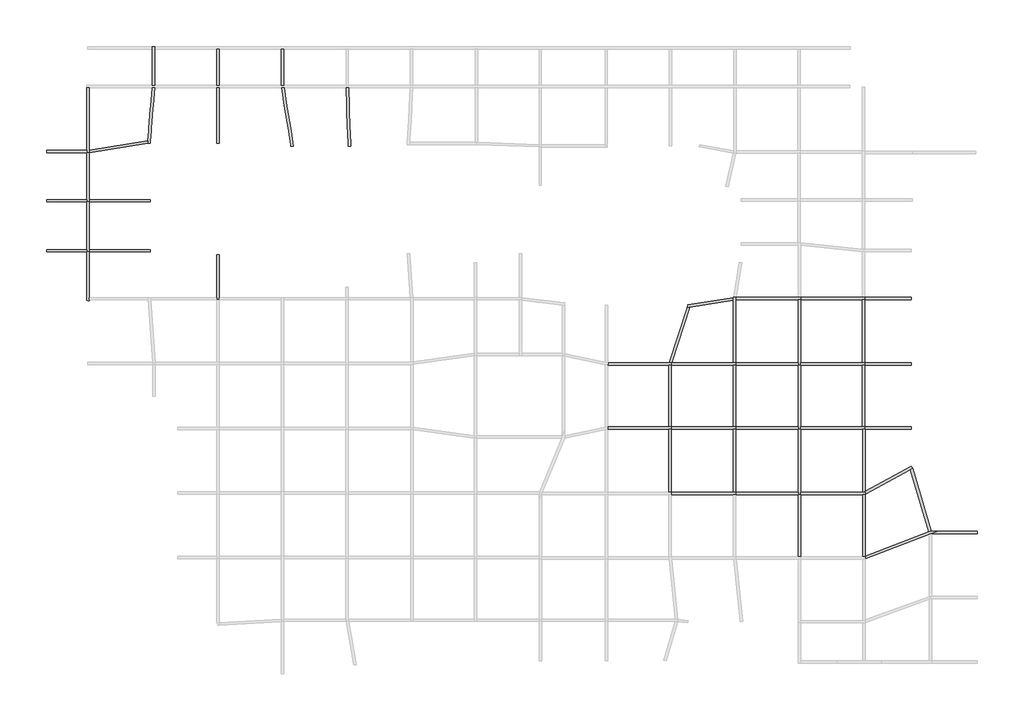
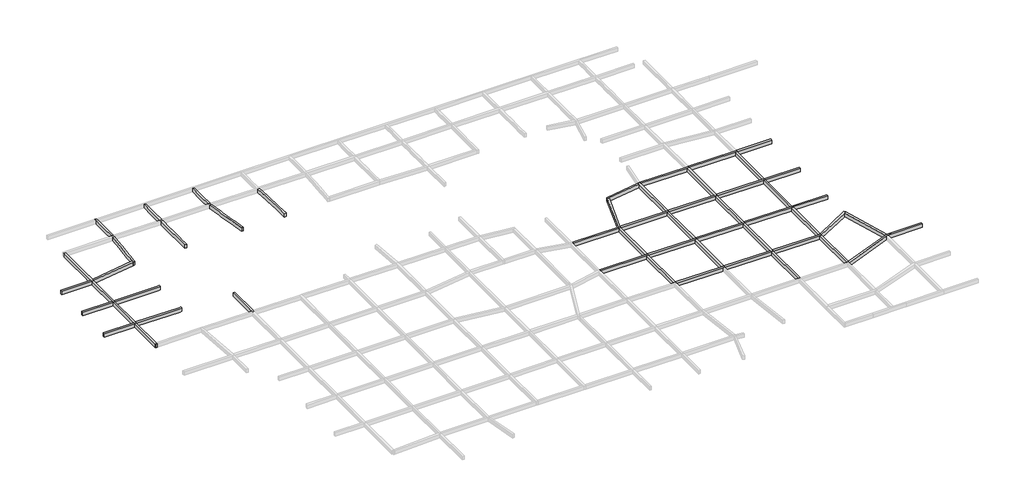
# One storey, part 6 of 8: 53 beams.
"""IFC4 building model written with IfcOpenShell, lengths in millimetres."""

from ifc_helpers import new_model, si_unit, frame, origin, place, context, project, spatial, polyline, outline, extrude, faceted_brep, element, save

model = new_model("IFC4")

# Units and contexts
model_context = context("Model", 3, world=origin())
ifc_project = project(units=[si_unit("LENGTHUNIT", "METRE", prefix="MILLI")], contexts=[model_context])

# Site, building, storey
site = spatial("IfcSite", under=ifc_project)
building = spatial("IfcBuilding", under=site)
storey = spatial("IfcBuildingStorey", under=building, Name="层高", Elevation=3300.0)

# Beams
placement = place(None, origin())
element("IfcBeam", 1, ObjectType="混凝土 - 矩形梁 : KL_beam", at=placement, inside=storey, context=model_context, shape_type="Brep", body=[
    faceted_brep([(62108.8476291, 145017.045189, 3300.0), (62408.8476291, 145017.045189, 3300.0), (62408.8476291, 145038.9496025, 3300.0), (62408.8476291, 145342.6952689, 3300.0), (62408.8476291, 147654.2446479, 3300.0), (62408.8476291, 148054.2446479, 3300.0), (62408.8476291, 150406.6496336, 3300.0), (62408.8476291, 150806.6496336, 3300.0), (62408.8476291, 152967.0451916, 3300.0), (62108.8476291, 152967.0451916, 3300.0), (62108.8476291, 145317.045189, 3300.0), (62108.8476291, 145017.045189, 2700.0), (62108.8476291, 152967.0451916, 2700.0), (62108.8476291, 150806.6496336, 2700.0), (62108.8476291, 150406.6496336, 2700.0), (62108.8476291, 148054.2446479, 2700.0), (62108.8476291, 147654.2446479, 2700.0), (62108.8476291, 145317.045189, 2700.0), (62408.8476291, 145017.045189, 2700.0), (62408.8476291, 152967.0451916, 2700.0), (62408.8476291, 150806.6496336, 2700.0), (62408.8476291, 150406.6496336, 2700.0), (62408.8476291, 148054.2446479, 2700.0), (62408.8476291, 147654.2446479, 2700.0), (62408.8476291, 145342.6952689, 2700.0), (62408.8476291, 145038.9496025, 2700.0)], [[[0, 1, 2, 3, 4, 5, 6, 7, 8, 9, 10]], [[11, 0, 10, 9, 12, 13, 14, 15, 16, 17]], [[18, 11, 17, 16, 15, 14, 13, 12, 19, 20, 21, 22, 23, 24, 25]], [[1, 18, 25, 24, 23, 22, 21, 20, 19, 8, 7, 6, 5, 4, 3, 2]], [[9, 8, 19, 12]], [[1, 0, 11, 18]]]),
])
element("IfcBeam", 2, ObjectType="混凝土 - 矩形梁 : KL_beam", at=placement, inside=storey, context=model_context, shape_type="SweptSolid", body=[
    extrude(outline(polyline([(57170.338145, 145017.045189), (57170.338145, 145317.045189), (62108.8476291, 145317.045189), (62108.8476291, 145017.045189), (57170.338145, 145017.045189)])), frame((0.0, 0.0, 2700.0), z_axis=(0.0, 0.0, 1.0), x_axis=(1.0, 0.0, 0.0)), (0.0, 0.0, 1.0), 600.0),
])
element("IfcBeam", 3, ObjectType="混凝土 - 矩形梁 : KL_beam", at=placement, inside=storey, context=model_context, shape_type="Brep", body=[
    faceted_brep([(62108.8476291, 139017.045189, 3300.0), (62408.8476291, 139017.045189, 3300.0), (62408.8476291, 139317.045189, 3300.0), (62408.8476291, 145017.045189, 3300.0), (62108.8476291, 145017.045189, 3300.0), (62108.8476291, 139317.045189, 3300.0), (62108.8476291, 139017.045189, 2700.0), (62108.8476291, 145017.045189, 2700.0), (62108.8476291, 139317.045189, 2700.0), (62408.8476291, 139017.045189, 2700.0), (62408.8476291, 145017.045189, 2700.0), (62408.8476291, 139317.045189, 2700.0)], [[[0, 1, 2, 3, 4, 5]], [[6, 0, 5, 4, 7, 8]], [[9, 6, 8, 7, 10, 11]], [[1, 9, 11, 10, 3, 2]], [[4, 3, 10, 7]], [[1, 0, 6, 9]]]),
])
element("IfcBeam", 4, ObjectType="混凝土 - 矩形梁 : KL_beam", at=placement, inside=storey, context=model_context, shape_type="Brep", body=[
    faceted_brep([(62108.8476291, 132904.2446453, 3300.0), (62408.8476291, 132904.2446453, 3300.0), (62408.8476291, 133204.2446453, 3300.0), (62408.8476291, 139017.045189, 3300.0), (62108.8476291, 139017.045189, 3300.0), (62108.8476291, 133204.2446453, 3300.0), (62108.8476291, 132904.2446453, 2700.0), (62108.8476291, 139017.045189, 2700.0), (62108.8476291, 133204.2446453, 2700.0), (62408.8476291, 132904.2446453, 2700.0), (62408.8476291, 139017.045189, 2700.0), (62408.8476291, 133204.2446453, 2700.0)], [[[0, 1, 2, 3, 4, 5]], [[6, 0, 5, 4, 7, 8]], [[9, 6, 8, 7, 10, 11]], [[1, 9, 11, 10, 3, 2]], [[1, 0, 6, 9]], [[4, 3, 10, 7]]]),
])
element("IfcBeam", 5, ObjectType="混凝土 - 矩形梁 : KL_beam", at=placement, inside=storey, context=model_context, shape_type="Brep", body=[
    faceted_brep([(62408.8476291, 126967.1449171, 2700.0), (62408.8476291, 126967.1449171, 3300.0), (62233.8430954, 126967.1449171, 3300.0), (62233.8430954, 126967.1449171, 2700.0), (62108.8476291, 127027.0451941, 3300.0), (62113.8430954, 127027.0451941, 3300.0), (62233.8430954, 127027.0451941, 3300.0), (62408.8476291, 127035.802002, 3300.0), (62408.8476291, 127335.802002, 3300.0), (62408.8476291, 132904.2446453, 3300.0), (62108.8476291, 132904.2446453, 3300.0), (62108.8476291, 127027.0451941, 2700.0), (62108.8476291, 132904.2446453, 2700.0), (62233.8430954, 127027.0451941, 2700.0), (62408.8476291, 132904.2446453, 2700.0), (62408.8476291, 127335.802002, 2700.0), (62408.8476291, 127035.802002, 2700.0)], [[[0, 1, 2, 3]], [[4, 5, 6, 2, 1, 7, 8, 9, 10]], [[11, 4, 10, 12]], [[13, 11, 12, 14, 15, 16, 0, 3]], [[1, 0, 16, 15, 14, 9, 8, 7]], [[4, 11, 13, 6, 5]], [[6, 13, 3, 2]], [[10, 9, 14, 12]]]),
])
element("IfcBeam", 6, ObjectType="混凝土 - 矩形梁 : KL_beam", at=placement, inside=storey, context=model_context, shape_type="SweptSolid", body=[
    extrude(outline(polyline([(57170.338145, 132904.2446453), (57170.338145, 133204.2446453), (62108.8476291, 133204.2446453), (62108.8476291, 132904.2446453), (57170.338145, 132904.2446453)])), frame((0.0, 0.0, 2700.0), z_axis=(0.0, 0.0, 1.0), x_axis=(1.0, 0.0, 0.0)), (0.0, 0.0, 1.0), 600.0),
])
element("IfcBeam", 7, ObjectType="混凝土 - 矩形梁 : KL_beam", at=placement, inside=storey, context=model_context, shape_type="SweptSolid", body=[
    extrude(outline(polyline([(57170.338145, 139017.045189), (57170.338145, 139317.045189), (62108.8476291, 139317.045189), (62108.8476291, 139017.045189), (57170.338145, 139017.045189)])), frame((0.0, 0.0, 2700.0), z_axis=(0.0, 0.0, 1.0), x_axis=(1.0, 0.0, 0.0)), (0.0, 0.0, 1.0), 600.0),
])
element("IfcBeam", 8, ObjectType="混凝土 - 矩形梁 : KL_beam", at=placement, inside=storey, context=model_context, shape_type="Brep", body=[
    faceted_brep([(70393.6976621, 158016.4462381, 3300.0), (70393.6976621, 158016.4462381, 2700.0), (70093.6976621, 158016.4462381, 2700.0), (70093.6976621, 158016.4462381, 3300.0), (70093.6976621, 158006.8472847, 3300.0), (70093.6976621, 157706.8472847, 3300.0), (70093.6976621, 155766.9462381, 3300.0), (70093.6976621, 155366.9462381, 3300.0), (70093.6976621, 153267.0451916, 3300.0), (70393.6976621, 153267.0451916, 3300.0), (70393.6976621, 155366.9462381, 3300.0), (70393.6976621, 155766.9462381, 3300.0), (70393.6976621, 157706.8472847, 3300.0), (70393.6976621, 158006.8472847, 3300.0), (70093.6976621, 158006.8472847, 2700.0), (70093.6976621, 157706.8472847, 2700.0), (70093.6976621, 155766.9462381, 2700.0), (70093.6976621, 155366.9462381, 2700.0), (70093.6976621, 153267.0451916, 2700.0), (70393.6976621, 158006.8472847, 2700.0), (70393.6976621, 157706.8472847, 2700.0), (70393.6976621, 155766.9462381, 2700.0), (70393.6976621, 155366.9462381, 2700.0), (70393.6976621, 153267.0451916, 2700.0)], [[[0, 1, 2, 3]], [[0, 3, 4, 5, 6, 7, 8, 9, 10, 11, 12, 13]], [[3, 2, 14, 15, 16, 17, 18, 8, 7, 6, 5, 4]], [[2, 1, 19, 20, 21, 22, 23, 18, 17, 16, 15, 14]], [[1, 0, 13, 12, 11, 10, 9, 23, 22, 21, 20, 19]], [[9, 8, 18, 23]]]),
])
element("IfcBeam", 9, ObjectType="混凝土 - 矩形梁 : KL_beam", at=placement, inside=storey, context=model_context, shape_type="Brep", body=[
    faceted_brep([(77972.7452463, 153267.0451916, 3300.0), (78272.7452463, 153267.0451916, 3300.0), (78272.7452463, 155366.9462381, 3300.0), (78272.7452463, 155766.9462381, 3300.0), (78272.7452463, 157706.8472847, 3300.0), (77972.7452463, 157706.8472847, 3300.0), (77972.7452463, 155766.9462381, 3300.0), (77972.7452463, 155366.9462381, 3300.0), (77972.7452463, 153267.0451916, 2700.0), (77972.7452463, 157706.8472847, 2700.0), (77972.7452463, 155766.9462381, 2700.0), (77972.7452463, 155366.9462381, 2700.0), (78272.7452463, 153267.0451916, 2700.0), (78272.7452463, 157706.8472847, 2700.0), (78272.7452463, 155766.9462381, 2700.0), (78272.7452463, 155366.9462381, 2700.0)], [[[0, 1, 2, 3, 4, 5, 6, 7]], [[8, 0, 7, 6, 5, 9, 10, 11]], [[12, 8, 11, 10, 9, 13, 14, 15]], [[1, 12, 15, 14, 13, 4, 3, 2]], [[1, 0, 8, 12]], [[5, 4, 13, 9]]]),
])
element("IfcBeam", 10, ObjectType="混凝土 - 矩形梁 : KL_beam", at=placement, inside=storey, context=model_context, shape_type="Brep", body=[
    faceted_brep([(85892.7452463, 153267.0451916, 3300.0), (86192.7452463, 153267.0451916, 3300.0), (86192.7452463, 155366.9462381, 3300.0), (86192.7452463, 155766.9462381, 3300.0), (86192.7452463, 157706.8472847, 3300.0), (85892.7452463, 157706.8472847, 3300.0), (85892.7452463, 155766.9462381, 3300.0), (85892.7452463, 155366.9462381, 3300.0), (85892.7452463, 153267.0451916, 2700.0), (85892.7452463, 157706.8472847, 2700.0), (85892.7452463, 155766.9462381, 2700.0), (85892.7452463, 155366.9462381, 2700.0), (86192.7452463, 153267.0451916, 2700.0), (86192.7452463, 157706.8472847, 2700.0), (86192.7452463, 155766.9462381, 2700.0), (86192.7452463, 155366.9462381, 2700.0)], [[[0, 1, 2, 3, 4, 5, 6, 7]], [[8, 0, 7, 6, 5, 9, 10, 11]], [[12, 8, 11, 10, 9, 13, 14, 15]], [[1, 12, 15, 14, 13, 4, 3, 2]], [[1, 0, 8, 12]], [[5, 4, 13, 9]]]),
])
element("IfcBeam", 11, ObjectType="混凝土 - 矩形梁 : KL_beam", at=placement, inside=storey, context=model_context, shape_type="Brep", body=[
    faceted_brep([(69518.4633077, 146165.9301761, 3300.0), (69533.6976621, 146168.3450494, 3300.0), (69695.5125279, 146193.9951293, 3300.0), (69823.484619, 146214.2806226, 3300.0), (69846.6115888, 146493.9951293, 3300.0), (69942.541742, 147654.2446479, 3300.0), (69975.6139913, 148054.2446479, 3300.0), (70170.1123015, 150406.6496336, 3300.0), (70203.1845508, 150806.6496336, 3300.0), (70381.8074018, 152967.0451916, 3300.0), (70080.7837355, 152967.0451916, 3300.0), (69902.1608844, 150806.6496336, 3300.0), (69869.0886352, 150406.6496336, 3300.0), (69674.590325, 148054.2446479, 3300.0), (69641.5180757, 147654.2446479, 3300.0), (69543.9107052, 146473.7096361, 3300.0), (69518.4633077, 146165.9301761, 2700.0), (70080.7837355, 152967.0451916, 2700.0), (69902.1608844, 150806.6496336, 2700.0), (69869.0886352, 150406.6496336, 2700.0), (69674.590325, 148054.2446479, 2700.0), (69641.5180757, 147654.2446479, 2700.0), (69543.9107052, 146473.7096361, 2700.0), (69823.484619, 146214.2806226, 2700.0), (69695.5125279, 146193.9951293, 2700.0), (69533.6976621, 146168.3450494, 2700.0), (70381.8074018, 152967.0451916, 2700.0), (70203.1845508, 150806.6496336, 2700.0), (70170.1123015, 150406.6496336, 2700.0), (69975.6139913, 148054.2446479, 2700.0), (69942.541742, 147654.2446479, 2700.0), (69846.6115888, 146493.9951293, 2700.0)], [[[0, 1, 2, 3, 4, 5, 6, 7, 8, 9, 10, 11, 12, 13, 14, 15]], [[16, 0, 15, 14, 13, 12, 11, 10, 17, 18, 19, 20, 21, 22]], [[23, 24, 25, 16, 22, 21, 20, 19, 18, 17, 26, 27, 28, 29, 30, 31]], [[3, 23, 31, 30, 29, 28, 27, 26, 9, 8, 7, 6, 5, 4]], [[10, 9, 26, 17]], [[3, 2, 1, 0, 16, 25, 24, 23]]]),
])
element("IfcBeam", 12, ObjectType="混凝土 - 矩形梁 : KL_beam", at=placement, inside=storey, context=model_context, shape_type="Brep", body=[
    faceted_brep([(62408.8476291, 145342.6952689, 2700.0), (62408.8476291, 145342.6952689, 3300.0), (69543.9107052, 146473.7096361, 3300.0), (69543.9107052, 146473.7096361, 2700.0), (62408.8476291, 145317.045189, 2700.0), (62408.8476291, 145038.9496025, 2700.0), (62408.8476291, 145038.9496025, 3300.0), (62408.8476291, 145317.045189, 3300.0), (69518.4633077, 146165.9301761, 3300.0), (69518.4633077, 146165.9301761, 2700.0)], [[[0, 1, 2, 3]], [[1, 0, 4, 5, 6, 7]], [[7, 6, 8, 2, 1]], [[4, 0, 3, 9, 5]], [[6, 5, 9, 8]], [[3, 2, 8, 9]]]),
])
element("IfcBeam", 13, ObjectType="混凝土 - 矩形梁 : KL_beam", at=placement, inside=storey, context=model_context, shape_type="Brep", body=[
    faceted_brep([(69858.8476291, 139317.045189, 3300.0), (69858.8476291, 139017.045189, 3300.0), (69858.8476291, 139017.045189, 2700.0), (69858.8476291, 139317.045189, 2700.0), (69833.6976621, 139317.045189, 3300.0), (69533.6976621, 139317.045189, 3300.0), (62408.8476291, 139317.045189, 3300.0), (62408.8476291, 139017.045189, 3300.0), (69533.6976621, 139017.045189, 3300.0), (69833.6976621, 139017.045189, 3300.0), (62408.8476291, 139017.045189, 2700.0), (69533.6976621, 139017.045189, 2700.0), (69833.6976621, 139017.045189, 2700.0), (62408.8476291, 139317.045189, 2700.0), (69533.6976621, 139317.045189, 2700.0), (69833.6976621, 139317.045189, 2700.0)], [[[0, 1, 2, 3]], [[1, 0, 4, 5, 6, 7, 8, 9]], [[2, 1, 9, 8, 7, 10, 11, 12]], [[3, 2, 12, 11, 10, 13, 14, 15]], [[0, 3, 15, 14, 13, 6, 5, 4]], [[7, 6, 13, 10]]]),
])
element("IfcBeam", 14, ObjectType="混凝土 - 矩形梁 : KL_beam", at=placement, inside=storey, context=model_context, shape_type="Brep", body=[
    faceted_brep([(69833.6976621, 132904.2446453, 3300.0), (69833.6976621, 133204.2446453, 3300.0), (69533.6976621, 133204.2446453, 3300.0), (62408.8476291, 133204.2446453, 3300.0), (62408.8476291, 132904.2446453, 3300.0), (69535.8470854, 132904.2446453, 3300.0), (69833.6976621, 132904.2446453, 2700.0), (62408.8476291, 132904.2446453, 2700.0), (69535.8470854, 132904.2446453, 2700.0), (69833.6976621, 133204.2446453, 2700.0), (62408.8476291, 133204.2446453, 2700.0), (69533.6976621, 133204.2446453, 2700.0)], [[[0, 1, 2, 3, 4, 5]], [[6, 0, 5, 4, 7, 8]], [[9, 6, 8, 7, 10, 11]], [[1, 9, 11, 10, 3, 2]], [[4, 3, 10, 7]], [[1, 0, 6, 9]]]),
])
element("IfcBeam", 15, ObjectType="混凝土 - 矩形梁 : KL_beam", at=placement, inside=storey, context=model_context, shape_type="Brep", body=[
    faceted_brep([(78292.6046485, 132543.8985649, 3300.0), (78292.6046485, 132543.8985649, 2700.0), (77992.6046485, 132543.8985649, 2700.0), (77992.6046485, 132543.8985649, 3300.0), (77992.6046485, 127335.802002, 3300.0), (77992.6046485, 127035.802002, 3300.0), (78270.8225114, 127035.802002, 3300.0), (78292.6046485, 127035.802002, 3300.0), (78292.6046485, 127335.802002, 3300.0), (77992.6046485, 127335.802002, 2700.0), (77992.6046485, 127035.802002, 2700.0), (78292.6046485, 127335.802002, 2700.0), (78292.6046485, 127035.802002, 2700.0), (78270.8225114, 127035.802002, 2700.0)], [[[0, 1, 2, 3]], [[0, 3, 4, 5, 6, 7, 8]], [[3, 2, 9, 10, 5, 4]], [[2, 1, 11, 12, 13, 10, 9]], [[1, 0, 8, 7, 12, 11]], [[7, 6, 5, 10, 13, 12]]]),
])
element("IfcBeam", 16, ObjectType="混凝土 - 矩形梁 : KL_beam", at=placement, inside=storey, context=model_context, shape_type="Brep", body=[
    faceted_brep([(125748.8238726, 111515.2247274, 3300.0), (125748.8238726, 111243.7571224, 3300.0), (125748.8238726, 111215.2247274, 3300.0), (133248.8238805, 111215.2247274, 3300.0), (133548.8238805, 111215.2247274, 3300.0), (133548.8238805, 111515.2247274, 3300.0), (133248.8238805, 111515.2247274, 3300.0), (133548.8238805, 111215.2247274, 2700.0), (125748.8238726, 111215.2247274, 2700.0), (133248.8238805, 111215.2247274, 2700.0), (125748.8238726, 111243.7571224, 2700.0), (125748.8238726, 111515.2247274, 2700.0), (133248.8238805, 111515.2247274, 2700.0), (133548.8238805, 111515.2247274, 2700.0)], [[[0, 1, 2, 3, 4, 5, 6]], [[7, 4, 3, 2, 8, 9]], [[8, 10, 11, 12, 13, 7, 9]], [[11, 0, 6, 5, 13, 12]], [[0, 11, 10, 8, 2, 1]], [[5, 4, 7, 13]]]),
])
element("IfcBeam", 17, ObjectType="混凝土 - 矩形梁 : KL_beam", at=placement, inside=storey, context=model_context, shape_type="Brep", body=[
    faceted_brep([(125814.5895158, 119344.1147453, 3300.0), (125783.0582452, 119044.1147453, 3300.0), (133248.8238805, 119044.1147453, 3300.0), (133548.8238805, 119044.1147453, 3300.0), (133548.8238805, 119344.1147453, 3300.0), (133289.6573621, 119344.1147453, 3300.0), (125783.0582452, 119044.1147453, 2700.0), (133248.8238805, 119044.1147453, 2700.0), (133548.8238805, 119044.1147453, 2700.0), (125814.5895158, 119344.1147453, 2700.0), (133289.6573621, 119344.1147453, 2700.0), (133548.8238805, 119344.1147453, 2700.0)], [[[0, 1, 2, 3, 4, 5]], [[1, 6, 7, 8, 3, 2]], [[6, 9, 10, 11, 8, 7]], [[9, 0, 5, 4, 11, 10]], [[0, 9, 6, 1]], [[4, 3, 8, 11]]]),
])
element("IfcBeam", 18, ObjectType="混凝土 - 矩形梁 : KL_beam", at=placement, inside=storey, context=model_context, shape_type="SweptSolid", body=[
    extrude(outline(polyline([(133548.8238805, 111515.2247274), (133248.8238805, 111515.2247274), (133248.8238805, 119044.1147453), (133548.8238805, 119044.1147453), (133548.8238805, 111515.2247274)])), frame((0.0, 0.0, 2700.0), z_axis=(0.0, 0.0, 1.0), x_axis=(1.0, 0.0, 0.0)), (0.0, 0.0, 1.0), 600.0),
])
element("IfcBeam", 19, ObjectType="混凝土 - 矩形梁 : KL_beam", at=placement, inside=storey, context=model_context, shape_type="SweptSolid", body=[
    extrude(outline(polyline([(133548.8238805, 103531.7102801), (133248.8238805, 103531.7102801), (133248.8238805, 111215.2247274), (133548.8238805, 111215.2247274), (133548.8238805, 103531.7102801)])), frame((0.0, 0.0, 2700.0), z_axis=(0.0, 0.0, 1.0), x_axis=(1.0, 0.0, 0.0)), (0.0, 0.0, 1.0), 600.0),
])
element("IfcBeam", 20, ObjectType="混凝土 - 矩形梁 : KL_beam", at=placement, inside=storey, context=model_context, shape_type="Brep", body=[
    faceted_brep([(141448.8238805, 119044.1147453, 3300.0), (141448.8238805, 119344.1147453, 3300.0), (141148.8238805, 119344.1147453, 3300.0), (133604.9310307, 119344.1147453, 3300.0), (133548.8238805, 119344.1147453, 3300.0), (133548.8238805, 119044.1147453, 3300.0), (141148.8238805, 119044.1147453, 3300.0), (141448.8238805, 119044.1147453, 2700.0), (133548.8238805, 119044.1147453, 2700.0), (141148.8238805, 119044.1147453, 2700.0), (141448.8238805, 119344.1147453, 2700.0), (133548.8238805, 119344.1147453, 2700.0), (133604.9310307, 119344.1147453, 2700.0), (141148.8238805, 119344.1147453, 2700.0)], [[[0, 1, 2, 3, 4, 5, 6]], [[7, 0, 6, 5, 8, 9]], [[10, 7, 9, 8, 11, 12, 13]], [[1, 10, 13, 12, 11, 4, 3, 2]], [[5, 4, 11, 8]], [[1, 0, 7, 10]]]),
])
element("IfcBeam", 21, ObjectType="混凝土 - 矩形梁 : KL_beam", at=placement, inside=storey, context=model_context, shape_type="Brep", body=[
    faceted_brep([(141448.8238805, 111215.2247274, 3300.0), (141448.8238805, 111515.2247274, 3300.0), (141148.8238805, 111515.2247274, 3300.0), (133548.8238805, 111515.2247274, 3300.0), (133548.8238805, 111215.2247274, 3300.0), (141148.8238805, 111215.2247274, 3300.0), (141448.8238805, 111215.2247274, 2700.0), (133548.8238805, 111215.2247274, 2700.0), (141148.8238805, 111215.2247274, 2700.0), (141448.8238805, 111515.2247274, 2700.0), (133548.8238805, 111515.2247274, 2700.0), (141148.8238805, 111515.2247274, 2700.0)], [[[0, 1, 2, 3, 4, 5]], [[6, 0, 5, 4, 7, 8]], [[9, 6, 8, 7, 10, 11]], [[1, 9, 11, 10, 3, 2]], [[4, 3, 10, 7]], [[1, 0, 6, 9]]]),
])
element("IfcBeam", 22, ObjectType="混凝土 - 矩形梁 : KL_beam", at=placement, inside=storey, context=model_context, shape_type="Brep", body=[
    faceted_brep([(141448.8238805, 103231.7102801, 3300.0), (141448.8238805, 103531.7102801, 3300.0), (141148.8238805, 103531.7102801, 3300.0), (133548.8238805, 103531.7102801, 3300.0), (133548.8238805, 103231.7102801, 3300.0), (141148.8238805, 103231.7102801, 3300.0), (141448.8238805, 103231.7102801, 2700.0), (133548.8238805, 103231.7102801, 2700.0), (141148.8238805, 103231.7102801, 2700.0), (141448.8238805, 103531.7102801, 2700.0), (133548.8238805, 103531.7102801, 2700.0), (141148.8238805, 103531.7102801, 2700.0)], [[[0, 1, 2, 3, 4, 5]], [[6, 0, 5, 4, 7, 8]], [[9, 6, 8, 7, 10, 11]], [[1, 9, 11, 10, 3, 2]], [[4, 3, 10, 7]], [[1, 0, 6, 9]]]),
])
element("IfcBeam", 23, ObjectType="混凝土 - 矩形梁 : KL_beam", at=placement, inside=storey, context=model_context, shape_type="SweptSolid", body=[
    extrude(outline(polyline([(141148.8238805, 111215.2247274), (141448.8238805, 111215.2247274), (141448.8238805, 103531.7102801), (141148.8238805, 103531.7102801), (141148.8238805, 111215.2247274)])), frame((0.0, 0.0, 2700.0), z_axis=(0.0, 0.0, 1.0), x_axis=(1.0, 0.0, 0.0)), (0.0, 0.0, 1.0), 600.0),
])
element("IfcBeam", 24, ObjectType="混凝土 - 矩形梁 : KL_beam", at=placement, inside=storey, context=model_context, shape_type="SweptSolid", body=[
    extrude(outline(polyline([(141148.8238805, 119044.1147453), (141448.8238805, 119044.1147453), (141448.8238805, 111515.2247274), (141148.8238805, 111515.2247274), (141148.8238805, 119044.1147453)])), frame((0.0, 0.0, 2700.0), z_axis=(0.0, 0.0, 1.0), x_axis=(1.0, 0.0, 0.0)), (0.0, 0.0, 1.0), 600.0),
])
element("IfcBeam", 25, ObjectType="混凝土 - 矩形梁 : KL_beam", at=placement, inside=storey, context=model_context, shape_type="Brep", body=[
    faceted_brep([(141448.8238805, 127344.1147453, 3300.0), (141170.7117777, 127344.1147453, 3300.0), (141148.8238805, 127344.1147453, 3300.0), (141148.8238805, 127321.9986816, 3300.0), (141148.8238805, 127205.9200013, 3300.0), (141148.8238805, 127018.1739614, 3300.0), (141148.8238805, 119344.1147453, 3300.0), (141448.8238805, 119344.1147453, 3300.0), (141448.8238805, 127044.1147453, 3300.0), (141448.8238805, 127344.1147453, 2700.0), (141448.8238805, 119344.1147453, 2700.0), (141448.8238805, 127044.1147453, 2700.0), (141148.8238805, 127344.1147453, 2700.0), (141170.7117777, 127344.1147453, 2700.0), (141148.8238805, 119344.1147453, 2700.0), (141148.8238805, 127018.1739614, 2700.0), (141148.8238805, 127205.9200013, 2700.0), (141148.8238805, 127321.9986816, 2700.0)], [[[0, 1, 2, 3, 4, 5, 6, 7, 8]], [[9, 0, 8, 7, 10, 11]], [[12, 13, 9, 11, 10, 14, 15, 16, 17]], [[2, 12, 17, 16, 15, 14, 6, 5, 4, 3]], [[7, 6, 14, 10]], [[2, 1, 0, 9, 13, 12]]]),
])
element("IfcBeam", 26, ObjectType="混凝土 - 矩形梁 : KL_beam", at=placement, inside=storey, context=model_context, shape_type="Brep", body=[
    faceted_brep([(149348.8238805, 127044.1147453, 3300.0), (149348.8238805, 127344.1147453, 3300.0), (149048.8238805, 127344.1147453, 3300.0), (141474.4513154, 127344.1147453, 3300.0), (141448.8238805, 127344.1147453, 3300.0), (141448.8238805, 127044.1147453, 3300.0), (149048.8238805, 127044.1147453, 3300.0), (149348.8238805, 127044.1147453, 2700.0), (141448.8238805, 127044.1147453, 2700.0), (149048.8238805, 127044.1147453, 2700.0), (149348.8238805, 127344.1147453, 2700.0), (141448.8238805, 127344.1147453, 2700.0), (141474.4513154, 127344.1147453, 2700.0), (149048.8238805, 127344.1147453, 2700.0)], [[[0, 1, 2, 3, 4, 5, 6]], [[7, 0, 6, 5, 8, 9]], [[10, 7, 9, 8, 11, 12, 13]], [[1, 10, 13, 12, 11, 4, 3, 2]], [[5, 4, 11, 8]], [[1, 0, 7, 10]]]),
])
element("IfcBeam", 27, ObjectType="混凝土 - 矩形梁 : KL_beam", at=placement, inside=storey, context=model_context, shape_type="Brep", body=[
    faceted_brep([(149048.8238805, 119044.1147453, 3300.0), (149348.8238805, 119044.1147453, 3300.0), (149348.8238805, 119344.1147453, 3300.0), (149348.8238805, 127044.1147453, 3300.0), (149048.8238805, 127044.1147453, 3300.0), (149048.8238805, 119344.1147453, 3300.0), (149048.8238805, 119044.1147453, 2700.0), (149048.8238805, 127044.1147453, 2700.0), (149048.8238805, 119344.1147453, 2700.0), (149348.8238805, 119044.1147453, 2700.0), (149348.8238805, 127044.1147453, 2700.0), (149348.8238805, 119344.1147453, 2700.0)], [[[0, 1, 2, 3, 4, 5]], [[6, 0, 5, 4, 7, 8]], [[9, 6, 8, 7, 10, 11]], [[1, 9, 11, 10, 3, 2]], [[4, 3, 10, 7]], [[1, 0, 6, 9]]]),
])
element("IfcBeam", 28, ObjectType="混凝土 - 矩形梁 : KL_beam", at=placement, inside=storey, context=model_context, shape_type="Brep", body=[
    faceted_brep([(149048.8238805, 111215.2247274, 3300.0), (149348.8238805, 111215.2247274, 3300.0), (149348.8238805, 111515.2247274, 3300.0), (149348.8238805, 119044.1147453, 3300.0), (149048.8238805, 119044.1147453, 3300.0), (149048.8238805, 111515.2247274, 3300.0), (149048.8238805, 111215.2247274, 2700.0), (149048.8238805, 119044.1147453, 2700.0), (149048.8238805, 111515.2247274, 2700.0), (149348.8238805, 111215.2247274, 2700.0), (149348.8238805, 119044.1147453, 2700.0), (149348.8238805, 111515.2247274, 2700.0)], [[[0, 1, 2, 3, 4, 5]], [[6, 0, 5, 4, 7, 8]], [[9, 6, 8, 7, 10, 11]], [[1, 9, 11, 10, 3, 2]], [[4, 3, 10, 7]], [[1, 0, 6, 9]]]),
])
element("IfcBeam", 29, ObjectType="混凝土 - 矩形梁 : KL_beam", at=placement, inside=storey, context=model_context, shape_type="SweptSolid", body=[
    extrude(outline(polyline([(141448.8238805, 119044.1147453), (141448.8238805, 119344.1147453), (149048.8238805, 119344.1147453), (149048.8238805, 119044.1147453), (141448.8238805, 119044.1147453)])), frame((0.0, 0.0, 2700.0), z_axis=(0.0, 0.0, 1.0), x_axis=(1.0, 0.0, 0.0)), (0.0, 0.0, 1.0), 600.0),
])
element("IfcBeam", 30, ObjectType="混凝土 - 矩形梁 : KL_beam", at=placement, inside=storey, context=model_context, shape_type="SweptSolid", body=[
    extrude(outline(polyline([(141448.8238805, 111215.2247274), (141448.8238805, 111515.2247274), (149048.8238805, 111515.2247274), (149048.8238805, 111215.2247274), (141448.8238805, 111215.2247274)])), frame((0.0, 0.0, 2700.0), z_axis=(0.0, 0.0, 1.0), x_axis=(1.0, 0.0, 0.0)), (0.0, 0.0, 1.0), 600.0),
])
element("IfcBeam", 31, ObjectType="混凝土 - 矩形梁 : KL_beam", at=placement, inside=storey, context=model_context, shape_type="Brep", body=[
    faceted_brep([(149048.8238805, 103231.7102801, 3300.0), (149348.8238805, 103231.7102801, 3300.0), (149348.8238805, 103531.7102801, 3300.0), (149348.8238805, 111215.2247274, 3300.0), (149048.8238805, 111215.2247274, 3300.0), (149048.8238805, 103531.7102801, 3300.0), (149048.8238805, 103231.7102801, 2700.0), (149048.8238805, 111215.2247274, 2700.0), (149048.8238805, 103531.7102801, 2700.0), (149348.8238805, 103231.7102801, 2700.0), (149348.8238805, 111215.2247274, 2700.0), (149348.8238805, 103531.7102801, 2700.0)], [[[0, 1, 2, 3, 4, 5]], [[6, 0, 5, 4, 7, 8]], [[9, 6, 8, 7, 10, 11]], [[1, 9, 11, 10, 3, 2]], [[4, 3, 10, 7]], [[1, 0, 6, 9]]]),
])
element("IfcBeam", 32, ObjectType="混凝土 - 矩形梁 : KL_beam", at=placement, inside=storey, context=model_context, shape_type="SweptSolid", body=[
    extrude(outline(polyline([(141448.8238805, 103231.7102801), (141448.8238805, 103531.7102801), (149048.8238805, 103531.7102801), (149048.8238805, 103231.7102801), (141448.8238805, 103231.7102801)])), frame((0.0, 0.0, 2700.0), z_axis=(0.0, 0.0, 1.0), x_axis=(1.0, 0.0, 0.0)), (0.0, 0.0, 1.0), 600.0),
])
element("IfcBeam", 33, ObjectType="混凝土 - 矩形梁 : KL_beam", at=placement, inside=storey, context=model_context, shape_type="SweptSolid", body=[
    extrude(outline(polyline([(149048.8238805, 103231.7102801), (149348.8238805, 103231.7102801), (149348.8238805, 95631.7102801), (149048.8238805, 95631.7102801), (149048.8238805, 103231.7102801)])), frame((0.0, 0.0, 2700.0), z_axis=(0.0, 0.0, 1.0), x_axis=(1.0, 0.0, 0.0)), (0.0, 0.0, 1.0), 600.0),
])
element("IfcBeam", 34, ObjectType="混凝土 - 矩形梁 : KL_beam", at=placement, inside=storey, context=model_context, shape_type="Brep", body=[
    faceted_brep([(157205.5468539, 127044.1147453, 3300.0), (157205.5468539, 127344.1147453, 3300.0), (156905.5468539, 127344.1147453, 3300.0), (149348.8238805, 127344.1147453, 3300.0), (149348.8238805, 127044.1147453, 3300.0), (156905.5468539, 127044.1147453, 3300.0), (157205.5468539, 127044.1147453, 2700.0), (149348.8238805, 127044.1147453, 2700.0), (156905.5468539, 127044.1147453, 2700.0), (157205.5468539, 127344.1147453, 2700.0), (149348.8238805, 127344.1147453, 2700.0), (156905.5468539, 127344.1147453, 2700.0)], [[[0, 1, 2, 3, 4, 5]], [[6, 0, 5, 4, 7, 8]], [[9, 6, 8, 7, 10, 11]], [[1, 9, 11, 10, 3, 2]], [[4, 3, 10, 7]], [[1, 0, 6, 9]]]),
])
element("IfcBeam", 35, ObjectType="混凝土 - 矩形梁 : KL_beam", at=placement, inside=storey, context=model_context, shape_type="SweptSolid", body=[
    extrude(outline(polyline([(162873.6972933, 127344.1147453), (162873.6972933, 127044.1147453), (157205.5468539, 127044.1147453), (157205.5468539, 127344.1147453), (162873.6972933, 127344.1147453)])), frame((0.0, 0.0, 2700.0), z_axis=(0.0, 0.0, 1.0), x_axis=(1.0, 0.0, 0.0)), (0.0, 0.0, 1.0), 600.0),
])
element("IfcBeam", 36, ObjectType="混凝土 - 矩形梁 : KL_beam", at=placement, inside=storey, context=model_context, shape_type="Brep", body=[
    faceted_brep([(157205.5468539, 119044.1147453, 3300.0), (157205.5468539, 119344.1147453, 3300.0), (156905.5468539, 119344.1147453, 3300.0), (149348.8238805, 119344.1147453, 3300.0), (149348.8238805, 119044.1147453, 3300.0), (156905.5468539, 119044.1147453, 3300.0), (157205.5468539, 119044.1147453, 2700.0), (149348.8238805, 119044.1147453, 2700.0), (156905.5468539, 119044.1147453, 2700.0), (157205.5468539, 119344.1147453, 2700.0), (149348.8238805, 119344.1147453, 2700.0), (156905.5468539, 119344.1147453, 2700.0)], [[[0, 1, 2, 3, 4, 5]], [[6, 0, 5, 4, 7, 8]], [[9, 6, 8, 7, 10, 11]], [[1, 9, 11, 10, 3, 2]], [[4, 3, 10, 7]], [[1, 0, 6, 9]]]),
])
element("IfcBeam", 37, ObjectType="混凝土 - 矩形梁 : KL_beam", at=placement, inside=storey, context=model_context, shape_type="SweptSolid", body=[
    extrude(outline(polyline([(162873.6972933, 119344.1147453), (162873.6972933, 119044.1147453), (157205.5468539, 119044.1147453), (157205.5468539, 119344.1147453), (162873.6972933, 119344.1147453)])), frame((0.0, 0.0, 2700.0), z_axis=(0.0, 0.0, 1.0), x_axis=(1.0, 0.0, 0.0)), (0.0, 0.0, 1.0), 600.0),
])
element("IfcBeam", 38, ObjectType="混凝土 - 矩形梁 : KL_beam", at=placement, inside=storey, context=model_context, shape_type="Brep", body=[
    faceted_brep([(157205.5468539, 111215.2247274, 3300.0), (157205.5468539, 111515.2247274, 3300.0), (156905.5468539, 111515.2247274, 3300.0), (149348.8238805, 111515.2247274, 3300.0), (149348.8238805, 111215.2247274, 3300.0), (156948.8238805, 111215.2247274, 3300.0), (157205.5468539, 111215.2247274, 2700.0), (149348.8238805, 111215.2247274, 2700.0), (156948.8238805, 111215.2247274, 2700.0), (157205.5468539, 111515.2247274, 2700.0), (149348.8238805, 111515.2247274, 2700.0), (156905.5468539, 111515.2247274, 2700.0)], [[[0, 1, 2, 3, 4, 5]], [[6, 0, 5, 4, 7, 8]], [[9, 6, 8, 7, 10, 11]], [[1, 9, 11, 10, 3, 2]], [[4, 3, 10, 7]], [[1, 0, 6, 9]]]),
])
element("IfcBeam", 39, ObjectType="混凝土 - 矩形梁 : KL_beam", at=placement, inside=storey, context=model_context, shape_type="Brep", body=[
    faceted_brep([(162873.6972933, 111515.2247274, 3300.0), (162873.6972933, 111215.2247274, 3300.0), (162873.6972933, 111215.2247274, 2700.0), (162873.6972933, 111515.2247274, 2700.0), (157205.5468539, 111515.2247274, 3300.0), (157205.5468539, 111215.2247274, 3300.0), (157248.8238805, 111215.2247274, 3300.0), (157205.5468539, 111215.2247274, 2700.0), (157248.8238805, 111215.2247274, 2700.0), (157205.5468539, 111515.2247274, 2700.0)], [[[0, 1, 2, 3]], [[1, 0, 4, 5, 6]], [[2, 1, 6, 5, 7, 8]], [[3, 2, 8, 7, 9]], [[0, 3, 9, 4]], [[5, 4, 9, 7]]]),
])
element("IfcBeam", 40, ObjectType="混凝土 - 矩形梁 : KL_beam", at=placement, inside=storey, context=model_context, shape_type="Brep", body=[
    faceted_brep([(157248.8238805, 103231.7102801, 3300.0), (157248.8238805, 103292.4607387, 3300.0), (157248.8238805, 103531.7102801, 3300.0), (157060.7357457, 103531.7102801, 3300.0), (156948.8238805, 103531.7102801, 3300.0), (149348.8238805, 103531.7102801, 3300.0), (149348.8238805, 103231.7102801, 3300.0), (156948.8238805, 103231.7102801, 3300.0), (157248.8238805, 103231.7102801, 2700.0), (149348.8238805, 103231.7102801, 2700.0), (156948.8238805, 103231.7102801, 2700.0), (157248.8238805, 103531.7102801, 2700.0), (157248.8238805, 103292.4607387, 2700.0), (149348.8238805, 103531.7102801, 2700.0), (156948.8238805, 103531.7102801, 2700.0), (157060.7357457, 103531.7102801, 2700.0)], [[[0, 1, 2, 3, 4, 5, 6, 7]], [[8, 0, 7, 6, 9, 10]], [[11, 12, 8, 10, 9, 13, 14, 15]], [[2, 11, 15, 14, 13, 5, 4, 3]], [[6, 5, 13, 9]], [[2, 1, 0, 8, 12, 11]]]),
])
element("IfcBeam", 41, ObjectType="混凝土 - 矩形梁 : KL_beam", at=placement, inside=storey, context=model_context, shape_type="Brep", body=[
    faceted_brep([(157248.8238805, 103231.7102801, 3300.0), (156948.8238805, 103231.7102801, 3300.0), (156948.8238805, 95631.7102801, 3300.0), (157248.8238805, 95631.7102801, 3300.0), (157248.8238805, 95699.9616344, 3300.0), (156948.8238805, 103231.7102801, 2700.0), (156948.8238805, 95631.7102801, 2700.0), (157248.8238805, 103231.7102801, 2700.0), (157248.8238805, 95699.9616344, 2700.0), (157248.8238805, 95631.7102801, 2700.0)], [[[0, 1, 2, 3, 4]], [[1, 5, 6, 2]], [[5, 7, 8, 9, 6]], [[7, 0, 4, 3, 9, 8]], [[1, 0, 7, 5]], [[3, 2, 6, 9]]]),
])
element("IfcBeam", 42, ObjectType="混凝土 - 矩形梁 : KL_beam", at=placement, inside=storey, context=model_context, shape_type="Brep", body=[
    faceted_brep([(157248.8238805, 95699.9616344, 3300.0), (157248.8238805, 95631.7102801, 3300.0), (157248.8238805, 95378.6181363, 3300.0), (165070.973591, 98381.2600869, 3300.0), (165248.7744478, 98449.5114412, 3300.0), (166030.3011672, 98749.5114412, 3300.0), (165332.9572274, 98749.5114412, 3300.0), (165193.1727343, 98749.5114412, 3300.0), (165037.7398112, 98689.8463321, 3300.0), (157248.8238805, 95378.6181363, 2700.0), (165070.973591, 98381.2600869, 2700.0), (165248.7744478, 98449.5114412, 2700.0), (166030.3011672, 98749.5114412, 2700.0), (157248.8238805, 95631.7102801, 2700.0), (157248.8238805, 95699.9616344, 2700.0), (165037.7398112, 98689.8463321, 2700.0), (165193.1727343, 98749.5114412, 2700.0), (165332.9572274, 98749.5114412, 2700.0)], [[[0, 1, 2, 3, 4, 5, 6, 7, 8]], [[2, 9, 10, 11, 12, 5, 4, 3]], [[9, 13, 14, 15, 16, 17, 12, 11, 10]], [[14, 0, 8, 7, 16, 15]], [[9, 2, 1, 0, 14, 13]], [[7, 6, 5, 12, 17, 16]]]),
])
element("IfcBeam", 43, ObjectType="混凝土 - 矩形梁 : KL_beam", at=placement, inside=storey, context=model_context, shape_type="Brep", body=[
    faceted_brep([(170973.3987408, 98749.5114412, 3300.0), (170973.3987408, 98449.5114412, 3300.0), (170973.3987408, 98449.5114412, 2700.0), (170973.3987408, 98749.5114412, 2700.0), (166030.3011672, 98749.5114412, 3300.0), (165248.7744478, 98449.5114412, 3300.0), (165370.973591, 98449.5114412, 3300.0), (165248.7744478, 98449.5114412, 2700.0), (165370.973591, 98449.5114412, 2700.0), (166030.3011672, 98749.5114412, 2700.0)], [[[0, 1, 2, 3]], [[1, 0, 4, 5, 6]], [[2, 1, 6, 5, 7, 8]], [[3, 2, 8, 7, 9]], [[0, 3, 9, 4]], [[5, 4, 9, 7]]]),
])
element("IfcBeam", 44, ObjectType="混凝土 - 矩形梁 : KL_beam", at=placement, inside=storey, context=model_context, shape_type="Brep", body=[
    faceted_brep([(162909.0729113, 106706.4332113, 3300.0), (157248.8238805, 103633.8124158, 3300.0), (157060.7357457, 103531.7102801, 3300.0), (157248.8238805, 103531.7102801, 3300.0), (157248.8238805, 103292.4607387, 3300.0), (162782.6675088, 106296.4633751, 3300.0), (163052.1973825, 106442.7755056, 3300.0), (157248.8238805, 103292.4607387, 2700.0), (162782.6675088, 106296.4633751, 2700.0), (163052.1973825, 106442.7755056, 2700.0), (157248.8238805, 103531.7102801, 2700.0), (157060.7357457, 103531.7102801, 2700.0), (157248.8238805, 103633.8124158, 2700.0), (162909.0729113, 106706.4332113, 2700.0)], [[[0, 1, 2, 3, 4, 5, 6]], [[6, 5, 4, 7, 8, 9]], [[9, 8, 7, 10, 11, 12, 13]], [[2, 1, 0, 13, 12, 11]], [[10, 3, 2, 11]], [[3, 10, 7, 4]], [[0, 6, 9, 13]]]),
])
element("IfcBeam", 45, ObjectType="混凝土 - 矩形梁 : KL_beam", at=placement, inside=storey, context=model_context, shape_type="Brep", body=[
    faceted_brep([(165332.9572274, 98749.5114412, 3300.0), (163052.1973825, 106442.7755056, 3300.0), (162782.6675088, 106296.4633751, 3300.0), (165037.7398112, 98689.8463321, 3300.0), (165070.973591, 98702.603585, 3300.0), (165193.1727343, 98749.5114412, 3300.0), (165332.9572274, 98749.5114412, 2700.0), (163052.1973825, 106442.7755056, 2700.0), (165193.1727343, 98749.5114412, 2700.0), (165070.973591, 98702.603585, 2700.0), (165037.7398112, 98689.8463321, 2700.0), (162782.6675088, 106296.4633751, 2700.0)], [[[0, 1, 2, 3, 4, 5]], [[1, 0, 6, 7]], [[7, 6, 8, 9, 10, 11]], [[10, 3, 2, 11]], [[8, 5, 4, 3, 10, 9]], [[5, 8, 6, 0]], [[2, 1, 7, 11]]]),
])
element("IfcBeam", 46, ObjectType="混凝土 - 矩形梁 : KL_beam", at=placement, inside=storey, context=model_context, shape_type="Brep", body=[
    faceted_brep([(135579.2996574, 126429.8194233, 3300.0), (135475.7638068, 126109.4093478, 3300.0), (135808.2478124, 126162.6697918, 3300.0), (141118.3137403, 127013.2865575, 3300.0), (141148.8238805, 127205.9200013, 3300.0), (141148.8238805, 127321.9986816, 3300.0), (141148.8238805, 127321.9986816, 2700.0), (135579.2996574, 126429.8194233, 2700.0), (135475.7638068, 126109.4093478, 2700.0), (141148.8238805, 127205.9200013, 2700.0), (141118.3137403, 127013.2865575, 2700.0), (135808.2478124, 126162.6697918, 2700.0)], [[[0, 1, 2, 3, 4, 5]], [[5, 6, 7, 0]], [[8, 7, 6, 9, 10, 11]], [[1, 8, 11, 10, 3, 2]], [[6, 5, 4, 9]], [[4, 3, 10, 9]], [[1, 0, 7, 8]]]),
])
element("IfcBeam", 47, ObjectType="混凝土 - 矩形梁 : KL_beam", at=placement, inside=storey, context=model_context, shape_type="Brep", body=[
    faceted_brep([(133289.6573621, 119344.1147453, 3300.0), (133548.8238805, 119344.1147453, 3300.0), (133604.9310307, 119344.1147453, 3300.0), (135808.2478124, 126162.6697918, 3300.0), (135475.7638068, 126109.4093478, 3300.0), (133289.6573621, 119344.1147453, 2700.0), (135475.7638068, 126109.4093478, 2700.0), (133604.9310307, 119344.1147453, 2700.0), (133548.8238805, 119344.1147453, 2700.0), (135808.2478124, 126162.6697918, 2700.0)], [[[0, 1, 2, 3, 4]], [[5, 0, 4, 6]], [[7, 8, 5, 6, 9]], [[2, 7, 9, 3]], [[0, 5, 8, 7, 2, 1]], [[4, 3, 9, 6]]]),
])
element("IfcBeam", 48, ObjectType="混凝土 - 矩形梁 : KL_beam", at=placement, inside=storey, context=model_context, shape_type="SweptSolid", body=[
    extrude(outline(polyline([(156905.5468539, 127044.1147453), (157205.5468539, 127044.1147453), (157205.5468539, 119344.1147453), (156905.5468539, 119344.1147453), (156905.5468539, 127044.1147453)])), frame((0.0, 0.0, 2700.0), z_axis=(0.0, 0.0, 1.0), x_axis=(1.0, 0.0, 0.0)), (0.0, 0.0, 1.0), 600.0),
])
element("IfcBeam", 49, ObjectType="混凝土 - 矩形梁 : KL_beam", at=placement, inside=storey, context=model_context, shape_type="SweptSolid", body=[
    extrude(outline(polyline([(156905.5468539, 119044.1147453), (157205.5468539, 119044.1147453), (157205.5468539, 111515.2247274), (156905.5468539, 111515.2247274), (156905.5468539, 119044.1147453)])), frame((0.0, 0.0, 2700.0), z_axis=(0.0, 0.0, 1.0), x_axis=(1.0, 0.0, 0.0)), (0.0, 0.0, 1.0), 600.0),
])
element("IfcBeam", 50, ObjectType="混凝土 - 矩形梁 : KL_beam", at=placement, inside=storey, context=model_context, shape_type="Brep", body=[
    faceted_brep([(157248.8238805, 111215.2247274, 3300.0), (157205.5468539, 111215.2247274, 3300.0), (156948.8238805, 111215.2247274, 3300.0), (156948.8238805, 103531.7102801, 3300.0), (157060.7357457, 103531.7102801, 3300.0), (157248.8238805, 103633.8124158, 3300.0), (157248.8238805, 111215.2247274, 2700.0), (157248.8238805, 103633.8124158, 2700.0), (156948.8238805, 111215.2247274, 2700.0), (157205.5468539, 111215.2247274, 2700.0), (157060.7357457, 103531.7102801, 2700.0), (156948.8238805, 103531.7102801, 2700.0)], [[[0, 1, 2, 3, 4, 5]], [[6, 0, 5, 7]], [[8, 9, 6, 7, 10, 11]], [[2, 8, 11, 3]], [[8, 2, 1, 0, 6, 9]], [[3, 11, 10, 4]], [[5, 4, 10, 7]]]),
])
element("IfcBeam", 51, ObjectType="混凝土 - 矩形梁 : KL_beam", at=placement, inside=storey, context=model_context, shape_type="Brep", body=[
    faceted_brep([(77972.7452463, 146193.9951293, 3300.0), (78272.7452463, 146193.9951293, 3300.0), (78272.7452463, 146485.9555292, 3300.0), (78272.7452463, 147654.2446479, 3300.0), (78272.7452463, 148054.2446479, 3300.0), (78272.7452463, 150406.6496336, 3300.0), (78272.7452463, 150806.6496336, 3300.0), (78272.7452463, 152967.0451916, 3300.0), (77972.7452463, 152967.0451916, 3300.0), (77972.7452463, 150806.6496336, 3300.0), (77972.7452463, 150406.6496336, 3300.0), (77972.7452463, 148054.2446479, 3300.0), (77972.7452463, 147654.2446479, 3300.0), (77972.7452463, 146493.9951293, 3300.0), (77972.7452463, 146193.9951293, 2700.0), (77972.7452463, 152967.0451916, 2700.0), (77972.7452463, 150806.6496336, 2700.0), (77972.7452463, 150406.6496336, 2700.0), (77972.7452463, 148054.2446479, 2700.0), (77972.7452463, 147654.2446479, 2700.0), (77972.7452463, 146493.9951293, 2700.0), (78272.7452463, 146193.9951293, 2700.0), (78272.7452463, 152967.0451916, 2700.0), (78272.7452463, 150806.6496336, 2700.0), (78272.7452463, 150406.6496336, 2700.0), (78272.7452463, 148054.2446479, 2700.0), (78272.7452463, 147654.2446479, 2700.0), (78272.7452463, 146485.9555292, 2700.0)], [[[0, 1, 2, 3, 4, 5, 6, 7, 8, 9, 10, 11, 12, 13]], [[14, 0, 13, 12, 11, 10, 9, 8, 15, 16, 17, 18, 19, 20]], [[21, 14, 20, 19, 18, 17, 16, 15, 22, 23, 24, 25, 26, 27]], [[1, 21, 27, 26, 25, 24, 23, 22, 7, 6, 5, 4, 3, 2]], [[8, 7, 22, 15]], [[1, 0, 14, 21]]]),
])
element("IfcBeam", 52, ObjectType="混凝土 - 矩形梁 : KL_beam", at=placement, inside=storey, context=model_context, shape_type="Brep", body=[
    faceted_brep([(87044.6832098, 145832.1898733, 3300.0), (87344.6832098, 145855.8003854, 3300.0), (87059.8376218, 147654.2446479, 3300.0), (86996.4838457, 148054.2446479, 3300.0), (86623.8994986, 150406.6496336, 3300.0), (86560.5457225, 150806.6496336, 3300.0), (86218.3726812, 152967.0451916, 3300.0), (85914.6331434, 152967.0451916, 3300.0), (86256.8061848, 150806.6496336, 3300.0), (86320.1599609, 150406.6496336, 3300.0), (86692.744308, 148054.2446479, 3300.0), (86756.0980841, 147654.2446479, 3300.0), (87017.4727846, 146003.9897368, 3300.0), (87044.6832098, 145832.1898733, 2700.0), (85914.6331434, 152967.0451916, 2700.0), (86256.8061848, 150806.6496336, 2700.0), (86320.1599609, 150406.6496336, 2700.0), (86692.744308, 148054.2446479, 2700.0), (86756.0980841, 147654.2446479, 2700.0), (87017.4727846, 146003.9897368, 2700.0), (87344.6832098, 145855.8003854, 2700.0), (86218.3726812, 152967.0451916, 2700.0), (86560.5457225, 150806.6496336, 2700.0), (86623.8994986, 150406.6496336, 2700.0), (86996.4838457, 148054.2446479, 2700.0), (87059.8376218, 147654.2446479, 2700.0)], [[[0, 1, 2, 3, 4, 5, 6, 7, 8, 9, 10, 11, 12]], [[13, 0, 12, 11, 10, 9, 8, 7, 14, 15, 16, 17, 18, 19]], [[20, 13, 19, 18, 17, 16, 15, 14, 21, 22, 23, 24, 25]], [[1, 20, 25, 24, 23, 22, 21, 6, 5, 4, 3, 2]], [[7, 6, 21, 14]], [[1, 0, 13, 20]]]),
])
element("IfcBeam", 53, ObjectType="混凝土 - 矩形梁 : KL_beam", at=placement, inside=storey, context=model_context, shape_type="Brep", body=[
    faceted_brep([(94336.7562099, 145849.4715609, 3300.0), (94036.9389618, 145839.0017118, 3300.0), (94036.9389618, 145839.0017118, 2700.0), (94336.7562099, 145849.4715609, 2700.0), (94273.732145, 147654.2446479, 3300.0), (94259.7638372, 148054.2446479, 3300.0), (94177.6160449, 150406.6496336, 3300.0), (94163.6477371, 150806.6496336, 3300.0), (94088.2050618, 152967.0451916, 3300.0), (93788.0221985, 152967.0451916, 3300.0), (93863.4648738, 150806.6496336, 3300.0), (93877.4331816, 150406.6496336, 3300.0), (93959.5809739, 148054.2446479, 3300.0), (93973.5492817, 147654.2446479, 3300.0), (93788.0221985, 152967.0451916, 2700.0), (93863.4648738, 150806.6496336, 2700.0), (93877.4331816, 150406.6496336, 2700.0), (93959.5809739, 148054.2446479, 2700.0), (93973.5492817, 147654.2446479, 2700.0), (94088.2050618, 152967.0451916, 2700.0), (94163.6477371, 150806.6496336, 2700.0), (94177.6160449, 150406.6496336, 2700.0), (94259.7638372, 148054.2446479, 2700.0), (94273.732145, 147654.2446479, 2700.0)], [[[0, 1, 2, 3]], [[1, 0, 4, 5, 6, 7, 8, 9, 10, 11, 12, 13]], [[2, 1, 13, 12, 11, 10, 9, 14, 15, 16, 17, 18]], [[3, 2, 18, 17, 16, 15, 14, 19, 20, 21, 22, 23]], [[0, 3, 23, 22, 21, 20, 19, 8, 7, 6, 5, 4]], [[9, 8, 19, 14]]]),
])

save(model, "model.ifc")

# Revit data of these elements
# Type "混凝土 - 矩形梁 : KL_beam"
#   Length [instance default] = 1524 mm
#   b = 300 mm
#   h = 600 mm
#   Structural Material [instance default] = 混凝土 - 现场浇注混凝土
#   Assembly Code = ""
# Elements 1, 2, 3, 4, 5, 6, 7, 8, 9, 10, 11, 12, 13, 14, 15, 16, 17, 18, 19, 20, 21, 22, 23, 24, 25, 26, 27, 28, 29, 30, 31, 32, 33, 34, 35, 36, 37, 38, 39, 40, 41, 42, 43, 44, 45, 46, 47, 48, 49, 50, 51, 52, 53 (IfcBeam, "混凝土 - 矩形梁 : KL_beam")
#   Comments = ""
#   Structural Material = none
#   Phase Created = 新构造
# Materials
#   "混凝土 - 现场浇注混凝土": class "混凝土", colour RGB 192 192 192, transparency 0
